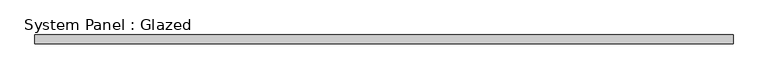
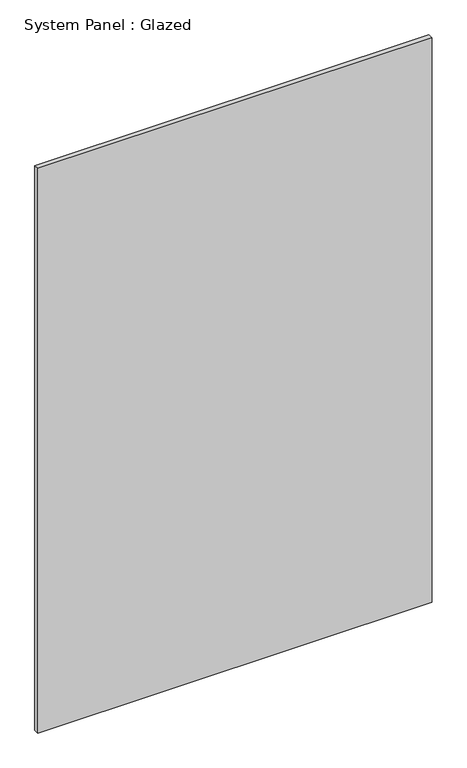
"""IFC4 building model written with IfcOpenShell, lengths in millimetres: plate geometry, System Panel : Glazed."""

import ifcopenshell
import ifcopenshell.guid

model = None  # the IFC model being written
_history = None  # IfcOwnerHistory: only IFC2X3 demands one
_inside = {}  # id of a spatial element -> (the spatial element, [elements in it])
_under = {}  # id of a project, library or spatial element -> (it, [spatial elements below it])
_declared = {}  # id of a project -> (the project, [libraries it declares])
_typed = {}  # id of a type object -> (the type object, [elements of that type])
_made_of = {}  # id of a material, layer set ... -> (it, [elements and type objects made of it])


def new_model(schema):
    """Start an empty IFC model of exactly this schema.

    Asked for "IFC4X3", IfcOpenShell would pick the latest addendum, in which some entities
    have other attributes; the version numbers below select the first issue.
    IFC2X3 requires an IfcOwnerHistory on every rooted entity: one is made here for all.
    """
    global model, _history
    if schema == "IFC4X3":
        model = ifcopenshell.file(schema_version=(4, 3, 0, 0))
    else:
        model = ifcopenshell.file(schema=schema)
    _inside.clear()
    _under.clear()
    _declared.clear()
    _typed.clear()
    _made_of.clear()
    _history = None
    if model.schema == "IFC2X3":
        org = make("IfcOrganization", Name="unknown")
        user = make(
            "IfcPersonAndOrganization",
            ThePerson=make("IfcPerson", FamilyName="unknown"),
            TheOrganization=org,
        )
        app = make(
            "IfcApplication",
            ApplicationDeveloper=org,
            Version="unknown",
            ApplicationFullName="unknown",
            ApplicationIdentifier="unknown",
        )
        _history = make(
            "IfcOwnerHistory",
            OwningUser=user,
            OwningApplication=app,
            ChangeAction="ADDED",
            CreationDate=0,
        )
    return model


def make(cls, **values):
    """One entity of the class cls with the attributes given. An attribute that is None is left unset."""
    return model.create_entity(
        cls, **{name: value for name, value in values.items() if value is not None}
    )


def rooted(cls, **values):
    """An entity with a GlobalId (a new one), such as an element, a storey or a relation."""
    return make(cls, GlobalId=ifcopenshell.guid.new(), OwnerHistory=_history, **values)


def si_unit(unit_type, name, prefix=None):
    """IfcSIUnit, for example si_unit("LENGTHUNIT", "METRE", prefix="MILLI")."""
    return make("IfcSIUnit", UnitType=unit_type, Prefix=prefix, Name=name)


def assignment(units):
    """IfcUnitAssignment: the units of a project."""
    return None if units is None else make("IfcUnitAssignment", Units=units)


def point(xyz):
    """IfcCartesianPoint."""
    return None if xyz is None else make("IfcCartesianPoint", Coordinates=xyz)


def direction(xyz):
    """IfcDirection."""
    return None if xyz is None else make("IfcDirection", DirectionRatios=xyz)


def frame(location, z_axis=None, x_axis=None):
    """IfcAxis2Placement3D, a coordinate frame: its origin and axes. An axis left out is left unset."""
    return make(
        "IfcAxis2Placement3D",
        Location=point(location),
        Axis=direction(z_axis),
        RefDirection=direction(x_axis),
    )


def origin():
    """The frame at (0, 0, 0) with its axes left unset."""
    return frame((0.0, 0.0, 0.0))


def origin_with_axes():
    """The frame at (0, 0, 0) with the z axis (0, 0, 1) and the x axis (1, 0, 0) written out."""
    return frame((0.0, 0.0, 0.0), z_axis=(0.0, 0.0, 1.0), x_axis=(1.0, 0.0, 0.0))


def place(relative_to, where):
    """IfcLocalPlacement: puts the frame where relative to a parent placement (None: the world)."""
    return make(
        "IfcLocalPlacement", PlacementRelTo=relative_to, RelativePlacement=where
    )


def context(
    kind, dimensions, precision=None, world=None, true_north=None, identifier=None
):
    """IfcGeometricRepresentationContext, for example the 3D "Model" context."""
    return make(
        "IfcGeometricRepresentationContext",
        ContextIdentifier=identifier,
        ContextType=kind,
        CoordinateSpaceDimension=dimensions,
        Precision=precision,
        WorldCoordinateSystem=world,
        TrueNorth=true_north,
    )


def project(units=None, contexts=None):
    """IfcProject with its units and contexts."""
    return rooted(
        "IfcProject",
        Name="project",
        RepresentationContexts=contexts,
        UnitsInContext=assignment(units),
    )


def spatial(cls, under=None, at=None, **own):
    """A site, building, storey or space (cls), placed at a placement, below another one or the project."""
    s = rooted(cls, ObjectPlacement=at, **own)
    if under is not None:
        _under.setdefault(under.id(), (under, []))[1].append(s)
    return s


def polyline(points):
    """IfcPolyline through the points."""
    return make("IfcPolyline", Points=[point(p) for p in points])


def outline(outer, holes=None, kind="AREA"):
    """IfcArbitraryClosedProfileDef: a profile drawn as a closed curve; with holes, ...WithVoids."""
    if holes is None:
        return make("IfcArbitraryClosedProfileDef", ProfileType=kind, OuterCurve=outer)
    return make(
        "IfcArbitraryProfileDefWithVoids",
        ProfileType=kind,
        OuterCurve=outer,
        InnerCurves=holes,
    )


def extrude(swept, where, along, depth):
    """IfcExtrudedAreaSolid: the profile swept, set in the frame where, extruded along a direction by depth."""
    return make(
        "IfcExtrudedAreaSolid",
        SweptArea=swept,
        Position=where,
        ExtrudedDirection=direction(along),
        Depth=depth,
    )


def shape(context_of_items, identifier, shape_type, items):
    """IfcShapeRepresentation: the items that make up one representation, for example the "Body"."""
    return make(
        "IfcShapeRepresentation",
        ContextOfItems=context_of_items,
        RepresentationIdentifier=identifier,
        RepresentationType=shape_type,
        Items=items,
    )


def source(mapping_origin, context_of_items, identifier, shape_type, items):
    """IfcRepresentationMap: a shape defined once, which mapped items show again and again."""
    return make(
        "IfcRepresentationMap",
        MappingOrigin=mapping_origin,
        MappedRepresentation=shape(context_of_items, identifier, shape_type, items),
    )


def transform(
    local_origin,
    x_axis=None,
    y_axis=None,
    z_axis=None,
    scale=None,
    scale2=None,
    scale3=None,
    uniform=True,
):
    """IfcCartesianTransformationOperator3D, or its non-uniform kind. x_axis, y_axis, z_axis: its Axis1, 2, 3."""
    if uniform:
        return make(
            "IfcCartesianTransformationOperator3D",
            Axis1=direction(x_axis),
            Axis2=direction(y_axis),
            LocalOrigin=point(local_origin),
            Scale=scale,
            Axis3=direction(z_axis),
        )
    return make(
        "IfcCartesianTransformationOperator3DnonUniform",
        Axis1=direction(x_axis),
        Axis2=direction(y_axis),
        LocalOrigin=point(local_origin),
        Scale=scale,
        Axis3=direction(z_axis),
        Scale2=scale2,
        Scale3=scale3,
    )


def mapped(mapping_source, mapping_target):
    """IfcMappedItem: shows the shape of a source again, moved by a transform."""
    return make(
        "IfcMappedItem", MappingSource=mapping_source, MappingTarget=mapping_target
    )


def made_of(thing, what):
    """Note that an element or type object is made of a material, layer set ...; save() writes the relation."""
    if what is not None:
        _made_of.setdefault(what.id(), (what, []))[1].append(thing)
    return thing


def element(
    cls,
    number,
    at=None,
    inside=None,
    cuts=None,
    type_object=None,
    material=None,
    context=None,
    identifier="Body",
    shape_type=None,
    held_by="IfcProductDefinitionShape",
    body=None,
    shapes=None,
    **own,
):
    """One element of the class cls, such as IfcWall. Its Tag is "e" and its number.

    at: its placement. inside: the storey or other place that contains it. cuts: it is an
    opening in that element (IfcRelVoidsElement). A single representation is given by context,
    identifier, shape_type and body (its items); several are given by shapes. held_by: the class
    of the entity that holds the representations. save() writes the other relations.
    """
    e = rooted(cls, Tag="e%d" % number, ObjectPlacement=at, **own)
    if body is not None:
        shapes = [shape(context, identifier, shape_type, body)]
    if shapes is not None:
        e.Representation = make(held_by, Representations=shapes)
    if inside is not None:
        _inside.setdefault(inside.id(), (inside, []))[1].append(e)
    if cuts is not None:
        rooted(
            "IfcRelVoidsElement", RelatingBuildingElement=cuts, RelatedOpeningElement=e
        )
    if type_object is not None:
        _typed.setdefault(type_object.id(), (type_object, []))[1].append(e)
    return made_of(e, material)


def aggregate(whole, parts):
    """IfcRelAggregates: a whole, such as a stair, and the parts it consists of."""
    return rooted("IfcRelAggregates", RelatingObject=whole, RelatedObjects=parts)


def save(model, path):
    """Write the relations noted so far, then the file.

    IfcRelAggregates (storeys below a building ...), IfcRelContainedInSpatialStructure (elements
    in a storey), IfcRelDefinesByType, IfcRelAssociatesMaterial and IfcRelDeclares: one each for
    every whole, place, type object, material and project.
    """
    for whole, parts in _under.values():
        aggregate(whole, parts)
    for where, things in _inside.values():
        rooted(
            "IfcRelContainedInSpatialStructure",
            RelatedElements=things,
            RelatingStructure=where,
        )
    for kind, things in _typed.values():
        rooted("IfcRelDefinesByType", RelatedObjects=things, RelatingType=kind)
    for what, things in _made_of.values():
        rooted("IfcRelAssociatesMaterial", RelatedObjects=things, RelatingMaterial=what)
    for by, libraries in _declared.values():
        rooted("IfcRelDeclares", RelatingContext=by, RelatedDefinitions=libraries)
    model.write(path)


def system_panel_glazed_c8490059(model_context):
    return source(origin(), model_context, "Body", "SweptSolid", [
        extrude(outline(polyline([(975.0, 24.5), (-975.0, 24.5), (-975.0, 49.5), (975.0, 49.5), (975.0, 24.5)])), origin_with_axes(), (0.0, 0.0, 1.0), 2950.0),
    ])


if __name__ == "__main__":
    model = new_model("IFC4")
    model_context = context("Model", 3, world=origin())
    ifc_project = project(units=[si_unit("LENGTHUNIT", "METRE", prefix="MILLI")], contexts=[model_context])
    site = spatial("IfcSite", under=ifc_project)
    building = spatial("IfcBuilding", under=site)
    placement = place(None, origin())
    system_panel_glazed_shape = system_panel_glazed_c8490059(model_context)
    element("IfcPlate", 1, ObjectType="System Panel : Glazed", at=placement, inside=building, context=model_context, shape_type="MappedRepresentation", body=[
        mapped(system_panel_glazed_shape, transform((0.0, 0.0, 0.0), x_axis=(1.0, 0.0, 0.0), y_axis=(0.0, 1.0, 0.0), z_axis=(0.0, 0.0, 1.0))),
    ])
    save(model, "model.ifc")

# Revit data of these elements
# Element 1 (IfcPlate, "System Panel : Glazed")
#   Materials on its faces: "Glass"
# Materials
#   "Glass": class "Glass", colour RGB 0 128 192, transparency 0.9
